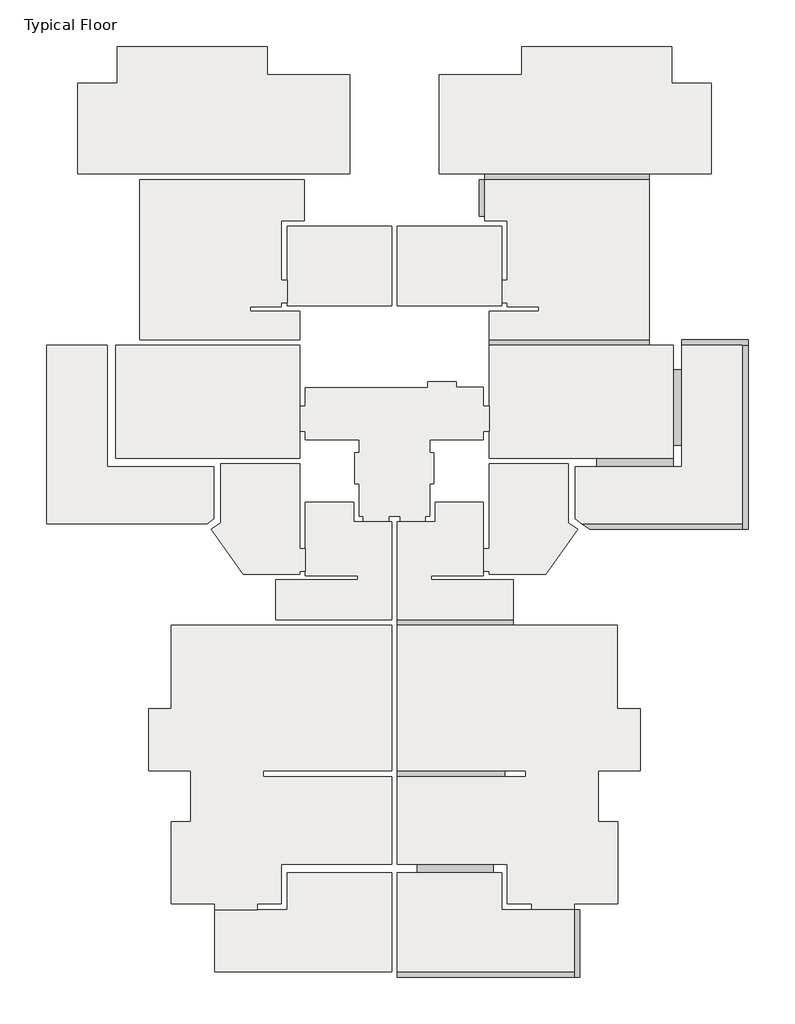
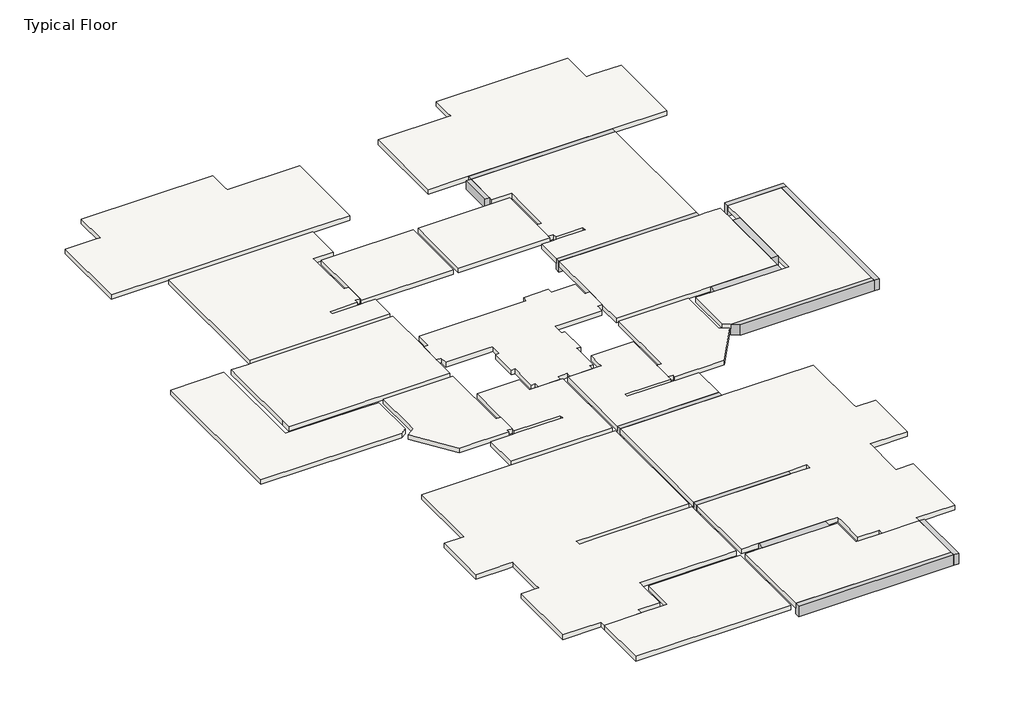
# One storey: 19 slabs, 13 beams.
# Revit data of these elements (continued)
# Element 5 (IfcBeam, "Concrete Rectengular Beam : 20/45") (continued)
#   Materials on its faces: "Concrete"
# Element 6 (IfcBeam, "Concrete Rectengular Beam : 20/45")
#   Comments = ""
#   Mark = "B17"
#   SOFiSTiK_AMG_Comments = ""
#   SOFiSTiK_AMG_Scheduled = yes
#   SOFiSTiK_AMG_Adjusted = yes
#   Structural Material = Concrete
#   Phase Created = New Construction
#   Materials on its faces: "Concrete"
# Element 7 (IfcBeam, "Concrete Rectengular Beam : 20/45")
#   Comments = ""
#   Mark = "B18"
#   SOFiSTiK_AMG_Comments = ""
#   SOFiSTiK_AMG_Scheduled = yes
#   SOFiSTiK_AMG_Adjusted = yes
#   Structural Material = Concrete
#   Phase Created = New Construction
#   Materials on its faces: "Concrete"
# Element 8 (IfcBeam, "Concrete Rectengular Beam : 20/45")
#   Comments = ""
#   Mark = "B20"
#   SOFiSTiK_AMG_Comments = ""
#   SOFiSTiK_AMG_Scheduled = yes
#   SOFiSTiK_AMG_Adjusted = yes
#   Structural Material = Concrete
#   Phase Created = New Construction
#   Materials on its faces: "Concrete"
# Element 9 (IfcBeam, "Concrete Rectengular Beam : 20/45")
#   Comments = ""
#   Mark = "B21"
#   SOFiSTiK_AMG_Comments = ""
#   SOFiSTiK_AMG_Scheduled = yes
#   SOFiSTiK_AMG_Adjusted = yes
#   Structural Material = Concrete
#   Phase Created = New Construction
#   Materials on its faces: "Concrete"
# Element 10 (IfcBeam, "Concrete Rectengular Beam : 20/45")
#   Comments = ""
#   Mark = "B22"
#   SOFiSTiK_AMG_Comments = ""
#   SOFiSTiK_AMG_Scheduled = yes
#   SOFiSTiK_AMG_Adjusted = yes
#   Structural Material = Concrete
#   Phase Created = New Construction
#   Materials on its faces: "Concrete"
# Element 11 (IfcBeam, "Concrete Rectengular Beam : 30/45")
#   Comments = ""
#   Mark = "B26"
#   SOFiSTiK_AMG_Comments = ""
#   SOFiSTiK_AMG_Scheduled = yes
#   SOFiSTiK_AMG_Adjusted = yes
#   Structural Material = Concrete
#   Phase Created = New Construction
#   Materials on its faces: "Concrete"
# Element 12 (IfcBeam, "Concrete Rectengular Beam : 30/45")
#   Comments = ""
#   Mark = "B27"
#   SOFiSTiK_AMG_Comments = ""
#   SOFiSTiK_AMG_Scheduled = yes
#   SOFiSTiK_AMG_Adjusted = yes
#   Structural Material = Concrete
#   Phase Created = New Construction
#   Materials on its faces: "Concrete"
# Element 13 (IfcBeam, "Concrete Rectengular Beam : 30/45")
#   Comments = ""
#   Mark = "B28"
#   SOFiSTiK_AMG_Comments = ""
#   SOFiSTiK_AMG_Scheduled = yes
#   SOFiSTiK_AMG_Adjusted = yes
#   Structural Material = Concrete
#   Phase Created = New Construction
#   Materials on its faces: "Concrete"
# Element 14 (IfcSlab, "20")
#   Mark = "S1"
#   SOFiSTiK_AMG_Comments = ""
#   built-in parameter 1001955 = 1.5708 (stored number, unit not read)
#   Height Offset From Level = 0 cm
#   built-in parameter 1001954 = 1
#   SOFiSTiK_AMG_Scheduled = yes
#   SOFiSTiK_AMG_Adjusted = yes
#   Phase Created = New Construction
#   Materials on its faces: "Concrete"
# Element 15 (IfcSlab, "20")
#   Mark = "S2"
#   SOFiSTiK_AMG_Comments = ""
#   built-in parameter 1001955 = 3.14159 (stored number, unit not read)
#   Height Offset From Level = 0 cm
#   built-in parameter 1001954 = 1
#   SOFiSTiK_AMG_Scheduled = yes
#   SOFiSTiK_AMG_Adjusted = yes
#   Phase Created = New Construction
#   Materials on its faces: "Concrete"
# Element 16 (IfcSlab, "20")
#   Mark = "S3"
#   SOFiSTiK_AMG_Comments = ""
#   built-in parameter 1001955 = 3.14159 (stored number, unit not read)
#   Height Offset From Level = 0 cm
#   built-in parameter 1001954 = 1
#   SOFiSTiK_AMG_Scheduled = yes
#   SOFiSTiK_AMG_Adjusted = yes
#   Phase Created = New Construction
#   Materials on its faces: "Concrete"
# Element 17 (IfcSlab, "20")
#   Mark = "S4"
#   SOFiSTiK_AMG_Comments = ""
#   Height Offset From Level = 0 cm
#   built-in parameter 1001954 = 1
#   SOFiSTiK_AMG_Scheduled = yes
#   SOFiSTiK_AMG_Adjusted = yes
#   Phase Created = New Construction
#   Materials on its faces: "Concrete"
# Element 18 (IfcSlab, "20")
#   Mark = "S5"
#   SOFiSTiK_AMG_Comments = ""
#   built-in parameter 1001955 = 3.14159 (stored number, unit not read)
#   Height Offset From Level = 0 cm
#   built-in parameter 1001954 = 1
#   SOFiSTiK_AMG_Scheduled = yes
#   SOFiSTiK_AMG_Adjusted = yes
#   Phase Created = New Construction
#   Materials on its faces: "Concrete"
# Element 19 (IfcSlab, "20")
#   Mark = "S6"
#   SOFiSTiK_AMG_Comments = ""
#   Height Offset From Level = 0 cm
#   built-in parameter 1001954 = 1
#   SOFiSTiK_AMG_Scheduled = yes
#   SOFiSTiK_AMG_Adjusted = yes
#   Phase Created = New Construction
#   Materials on its faces: "Concrete"
# Element 20 (IfcSlab, "20")
#   Mark = "S7"
#   SOFiSTiK_AMG_Comments = ""
#   built-in parameter 1001955 = 1.5708 (stored number, unit not read)
#   Height Offset From Level = 0 cm
#   built-in parameter 1001954 = 1
#   SOFiSTiK_AMG_Scheduled = yes
#   SOFiSTiK_AMG_Adjusted = yes
#   Phase Created = New Construction
#   Materials on its faces: "Concrete"
# Element 21 (IfcSlab, "20")
#   Mark = "S8"
#   SOFiSTiK_AMG_Comments = ""
#   Height Offset From Level = 0 cm
#   built-in parameter 1001954 = 1
#   SOFiSTiK_AMG_Scheduled = yes
#   SOFiSTiK_AMG_Adjusted = yes
#   Phase Created = New Construction
#   Materials on its faces: "Concrete"
# Element 22 (IfcSlab, "20")
#   Mark = "S9"
#   SOFiSTiK_AMG_Comments = ""
#   Height Offset From Level = 0 cm
#   built-in parameter 1001954 = 1
#   SOFiSTiK_AMG_Scheduled = yes
#   SOFiSTiK_AMG_Adjusted = yes
#   Phase Created = New Construction
#   Materials on its faces: "Concrete"
# Element 23 (IfcSlab, "20")
#   Mark = "S10"
#   SOFiSTiK_AMG_Comments = ""
#   built-in parameter 1001955 = 1.5708 (stored number, unit not read)
#   Height Offset From Level = 0 cm
#   built-in parameter 1001954 = 1
#   SOFiSTiK_AMG_Scheduled = yes
#   SOFiSTiK_AMG_Adjusted = yes
#   Phase Created = New Construction
#   Materials on its faces: "Concrete"
# Element 24 (IfcSlab, "20")
#   Mark = "S11"
#   SOFiSTiK_AMG_Comments = ""
#   built-in parameter 1001955 = 0 (stored number, unit not read)
#   Height Offset From Level = 0 cm
#   built-in parameter 1001954 = 1
#   SOFiSTiK_AMG_Scheduled = yes
#   SOFiSTiK_AMG_Adjusted = no
#   Phase Created = New Construction
#   Materials on its faces: "Concrete"
# Element 25 (IfcSlab, "20")
#   Mark = "S12"
#   SOFiSTiK_AMG_Comments = ""
#   built-in parameter 1001955 = 0 (stored number, unit not read)
#   Height Offset From Level = 0 cm
#   built-in parameter 1001954 = 1
#   SOFiSTiK_AMG_Scheduled = yes
#   SOFiSTiK_AMG_Adjusted = yes
#   Phase Created = New Construction
#   Materials on its faces: "Concrete"
# Element 26 (IfcSlab, "20")
#   Mark = "S13"
#   SOFiSTiK_AMG_Comments = ""
#   built-in parameter 1001955 = 3.14159 (stored number, unit not read)
#   Height Offset From Level = 0 cm
#   built-in parameter 1001954 = 1
#   SOFiSTiK_AMG_Scheduled = yes
#   SOFiSTiK_AMG_Adjusted = yes
#   Phase Created = New Construction
#   Materials on its faces: "Concrete"
# Element 27 (IfcSlab, "20")
#   Mark = "S14"
#   SOFiSTiK_AMG_Comments = ""
#   built-in parameter 1001955 = 0 (stored number, unit not read)
#   Height Offset From Level = 0 cm
#   built-in parameter 1001954 = 1
#   SOFiSTiK_AMG_Scheduled = yes
#   SOFiSTiK_AMG_Adjusted = yes
#   Phase Created = New Construction
#   Materials on its faces: "Concrete"
# Element 28 (IfcSlab, "20")
#   Mark = "S15"
#   SOFiSTiK_AMG_Comments = ""
#   built-in parameter 1001955 = 3.14159 (stored number, unit not read)
#   Height Offset From Level = 0 cm
#   built-in parameter 1001954 = 1
#   SOFiSTiK_AMG_Scheduled = yes
#   SOFiSTiK_AMG_Adjusted = yes
#   Phase Created = New Construction
#   Materials on its faces: "Concrete"
# Element 29 (IfcSlab, "20")
#   Mark = "S16"
#   SOFiSTiK_AMG_Comments = ""
#   built-in parameter 1001955 = 1.5708 (stored number, unit not read)
#   Height Offset From Level = 0 cm
#   built-in parameter 1001954 = 1
#   SOFiSTiK_AMG_Scheduled = yes
#   SOFiSTiK_AMG_Adjusted = yes
#   Phase Created = New Construction
#   Materials on its faces: "Concrete"
# Element 30 (IfcSlab, "20")
#   Mark = "S17"
#   SOFiSTiK_AMG_Comments = ""
#   built-in parameter 1001955 = 3.14159 (stored number, unit not read)
#   Height Offset From Level = 0 cm
#   built-in parameter 1001954 = 1
#   SOFiSTiK_AMG_Scheduled = yes
#   SOFiSTiK_AMG_Adjusted = yes
#   Phase Created = New Construction
#   Materials on its faces: "Concrete"
# Element 31 (IfcSlab, "20")
#   Mark = "S18"
#   SOFiSTiK_AMG_Comments = ""
#   built-in parameter 1001955 = 3.14159 (stored number, unit not read)
#   Height Offset From Level = 0 cm
#   built-in parameter 1001954 = 1
#   SOFiSTiK_AMG_Scheduled = yes
#   SOFiSTiK_AMG_Adjusted = yes
#   Phase Created = New Construction
#   Materials on its faces: "Concrete"
# Element 32 (IfcSlab, "20")
#   Mark = "S19"
#   SOFiSTiK_AMG_Comments = ""
#   built-in parameter 1001955 = 1.5708 (stored number, unit not read)
#   Height Offset From Level = 0 cm
#   built-in parameter 1001954 = 1
#   SOFiSTiK_AMG_Scheduled = yes
#   SOFiSTiK_AMG_Adjusted = yes
#   Phase Created = New Construction
#   Materials on its faces: "Concrete"
# Materials
#   "Concrete": class "Concrete", colour RGB 192 192 192, transparency 0, Keynote = "01000", Description = "Cast-in-place concrete", Cost = 0
